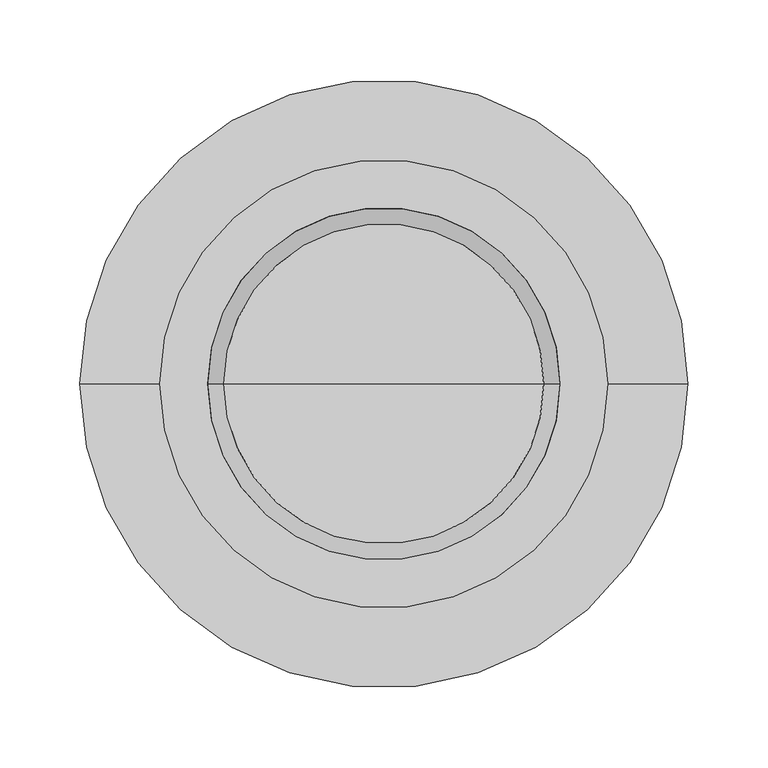
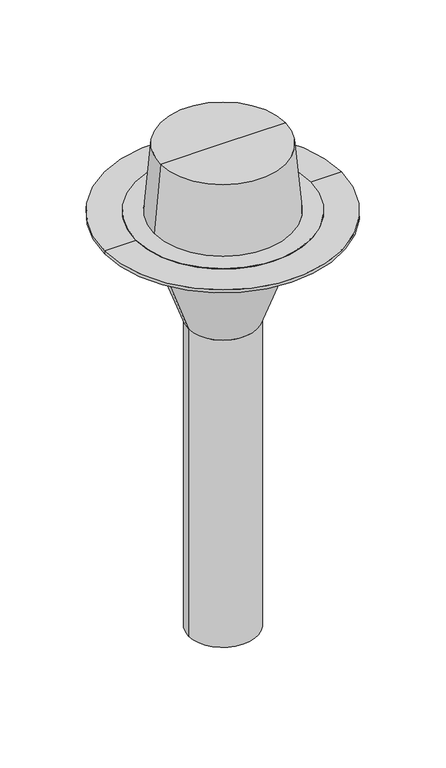
"""IFC4 building model written with IfcOpenShell, lengths in millimetres: proxy geometry, TN_Воронка ТехноНИКОЛЬ ЭКО : Воронка ТехноНИКОЛЬ ЭКО с обжимным фланцем Ø110х700мм."""

import ifcopenshell
import ifcopenshell.guid

model = None  # the IFC model being written
_history = None  # IfcOwnerHistory: only IFC2X3 demands one
_inside = {}  # id of a spatial element -> (the spatial element, [elements in it])
_under = {}  # id of a project, library or spatial element -> (it, [spatial elements below it])
_declared = {}  # id of a project -> (the project, [libraries it declares])
_typed = {}  # id of a type object -> (the type object, [elements of that type])
_made_of = {}  # id of a material, layer set ... -> (it, [elements and type objects made of it])


def new_model(schema):
    """Start an empty IFC model of exactly this schema.

    Asked for "IFC4X3", IfcOpenShell would pick the latest addendum, in which some entities
    have other attributes; the version numbers below select the first issue.
    IFC2X3 requires an IfcOwnerHistory on every rooted entity: one is made here for all.
    """
    global model, _history
    if schema == "IFC4X3":
        model = ifcopenshell.file(schema_version=(4, 3, 0, 0))
    else:
        model = ifcopenshell.file(schema=schema)
    _inside.clear()
    _under.clear()
    _declared.clear()
    _typed.clear()
    _made_of.clear()
    _history = None
    if model.schema == "IFC2X3":
        org = make("IfcOrganization", Name="unknown")
        user = make(
            "IfcPersonAndOrganization",
            ThePerson=make("IfcPerson", FamilyName="unknown"),
            TheOrganization=org,
        )
        app = make(
            "IfcApplication",
            ApplicationDeveloper=org,
            Version="unknown",
            ApplicationFullName="unknown",
            ApplicationIdentifier="unknown",
        )
        _history = make(
            "IfcOwnerHistory",
            OwningUser=user,
            OwningApplication=app,
            ChangeAction="ADDED",
            CreationDate=0,
        )
    return model


def make(cls, **values):
    """One entity of the class cls with the attributes given. An attribute that is None is left unset."""
    return model.create_entity(
        cls, **{name: value for name, value in values.items() if value is not None}
    )


def rooted(cls, **values):
    """An entity with a GlobalId (a new one), such as an element, a storey or a relation."""
    return make(cls, GlobalId=ifcopenshell.guid.new(), OwnerHistory=_history, **values)


def si_unit(unit_type, name, prefix=None):
    """IfcSIUnit, for example si_unit("LENGTHUNIT", "METRE", prefix="MILLI")."""
    return make("IfcSIUnit", UnitType=unit_type, Prefix=prefix, Name=name)


def assignment(units):
    """IfcUnitAssignment: the units of a project."""
    return None if units is None else make("IfcUnitAssignment", Units=units)


def point(xyz):
    """IfcCartesianPoint."""
    return None if xyz is None else make("IfcCartesianPoint", Coordinates=xyz)


def direction(xyz):
    """IfcDirection."""
    return None if xyz is None else make("IfcDirection", DirectionRatios=xyz)


def frame(location, z_axis=None, x_axis=None):
    """IfcAxis2Placement3D, a coordinate frame: its origin and axes. An axis left out is left unset."""
    return make(
        "IfcAxis2Placement3D",
        Location=point(location),
        Axis=direction(z_axis),
        RefDirection=direction(x_axis),
    )


def frame_2d(location, x_axis=None):
    """IfcAxis2Placement2D, a coordinate frame in the plane: its origin and x axis."""
    return make(
        "IfcAxis2Placement2D", Location=point(location), RefDirection=direction(x_axis)
    )


def origin():
    """The frame at (0, 0, 0) with its axes left unset."""
    return frame((0.0, 0.0, 0.0))


def origin_with_axes():
    """The frame at (0, 0, 0) with the z axis (0, 0, 1) and the x axis (1, 0, 0) written out."""
    return frame((0.0, 0.0, 0.0), z_axis=(0.0, 0.0, 1.0), x_axis=(1.0, 0.0, 0.0))


def origin_2d():
    """The frame at (0, 0) in the plane with its x axis left unset."""
    return frame_2d((0.0, 0.0))


def place(relative_to, where):
    """IfcLocalPlacement: puts the frame where relative to a parent placement (None: the world)."""
    return make(
        "IfcLocalPlacement", PlacementRelTo=relative_to, RelativePlacement=where
    )


def context(
    kind, dimensions, precision=None, world=None, true_north=None, identifier=None
):
    """IfcGeometricRepresentationContext, for example the 3D "Model" context."""
    return make(
        "IfcGeometricRepresentationContext",
        ContextIdentifier=identifier,
        ContextType=kind,
        CoordinateSpaceDimension=dimensions,
        Precision=precision,
        WorldCoordinateSystem=world,
        TrueNorth=true_north,
    )


def project(units=None, contexts=None):
    """IfcProject with its units and contexts."""
    return rooted(
        "IfcProject",
        Name="project",
        RepresentationContexts=contexts,
        UnitsInContext=assignment(units),
    )


def spatial(cls, under=None, at=None, **own):
    """A site, building, storey or space (cls), placed at a placement, below another one or the project."""
    s = rooted(cls, ObjectPlacement=at, **own)
    if under is not None:
        _under.setdefault(under.id(), (under, []))[1].append(s)
    return s


def polyline(points):
    """IfcPolyline through the points."""
    return make("IfcPolyline", Points=[point(p) for p in points])


def circle_curve(where, radius):
    """IfcCircle in the frame where."""
    return make("IfcCircle", Position=where, Radius=radius)


def trimmed(basis, trim1, trim2, sense, master):
    """IfcTrimmedCurve: the piece of a basis curve between two trims."""
    return make(
        "IfcTrimmedCurve",
        BasisCurve=basis,
        Trim1=trim1,
        Trim2=trim2,
        SenseAgreement=sense,
        MasterRepresentation=master,
    )


def segment(curve, same_sense, transition):
    """IfcCompositeCurveSegment."""
    return make(
        "IfcCompositeCurveSegment",
        Transition=transition,
        SameSense=same_sense,
        ParentCurve=curve,
    )


def composite_curve(segments, self_intersect=None):
    """IfcCompositeCurve: segments joined end to end."""
    return make("IfcCompositeCurve", Segments=segments, SelfIntersect=self_intersect)


def outline(outer, holes=None, kind="AREA"):
    """IfcArbitraryClosedProfileDef: a profile drawn as a closed curve; with holes, ...WithVoids."""
    if holes is None:
        return make("IfcArbitraryClosedProfileDef", ProfileType=kind, OuterCurve=outer)
    return make(
        "IfcArbitraryProfileDefWithVoids",
        ProfileType=kind,
        OuterCurve=outer,
        InnerCurves=holes,
    )


def extrude(swept, where, along, depth):
    """IfcExtrudedAreaSolid: the profile swept, set in the frame where, extruded along a direction by depth."""
    return make(
        "IfcExtrudedAreaSolid",
        SweptArea=swept,
        Position=where,
        ExtrudedDirection=direction(along),
        Depth=depth,
    )


def shape(context_of_items, identifier, shape_type, items):
    """IfcShapeRepresentation: the items that make up one representation, for example the "Body"."""
    return make(
        "IfcShapeRepresentation",
        ContextOfItems=context_of_items,
        RepresentationIdentifier=identifier,
        RepresentationType=shape_type,
        Items=items,
    )


def source(mapping_origin, context_of_items, identifier, shape_type, items):
    """IfcRepresentationMap: a shape defined once, which mapped items show again and again."""
    return make(
        "IfcRepresentationMap",
        MappingOrigin=mapping_origin,
        MappedRepresentation=shape(context_of_items, identifier, shape_type, items),
    )


def transform(
    local_origin,
    x_axis=None,
    y_axis=None,
    z_axis=None,
    scale=None,
    scale2=None,
    scale3=None,
    uniform=True,
):
    """IfcCartesianTransformationOperator3D, or its non-uniform kind. x_axis, y_axis, z_axis: its Axis1, 2, 3."""
    if uniform:
        return make(
            "IfcCartesianTransformationOperator3D",
            Axis1=direction(x_axis),
            Axis2=direction(y_axis),
            LocalOrigin=point(local_origin),
            Scale=scale,
            Axis3=direction(z_axis),
        )
    return make(
        "IfcCartesianTransformationOperator3DnonUniform",
        Axis1=direction(x_axis),
        Axis2=direction(y_axis),
        LocalOrigin=point(local_origin),
        Scale=scale,
        Axis3=direction(z_axis),
        Scale2=scale2,
        Scale3=scale3,
    )


def mapped(mapping_source, mapping_target):
    """IfcMappedItem: shows the shape of a source again, moved by a transform."""
    return make(
        "IfcMappedItem", MappingSource=mapping_source, MappingTarget=mapping_target
    )


def made_of(thing, what):
    """Note that an element or type object is made of a material, layer set ...; save() writes the relation."""
    if what is not None:
        _made_of.setdefault(what.id(), (what, []))[1].append(thing)
    return thing


def element(
    cls,
    number,
    at=None,
    inside=None,
    cuts=None,
    type_object=None,
    material=None,
    context=None,
    identifier="Body",
    shape_type=None,
    held_by="IfcProductDefinitionShape",
    body=None,
    shapes=None,
    **own,
):
    """One element of the class cls, such as IfcWall. Its Tag is "e" and its number.

    at: its placement. inside: the storey or other place that contains it. cuts: it is an
    opening in that element (IfcRelVoidsElement). A single representation is given by context,
    identifier, shape_type and body (its items); several are given by shapes. held_by: the class
    of the entity that holds the representations. save() writes the other relations.
    """
    e = rooted(cls, Tag="e%d" % number, ObjectPlacement=at, **own)
    if body is not None:
        shapes = [shape(context, identifier, shape_type, body)]
    if shapes is not None:
        e.Representation = make(held_by, Representations=shapes)
    if inside is not None:
        _inside.setdefault(inside.id(), (inside, []))[1].append(e)
    if cuts is not None:
        rooted(
            "IfcRelVoidsElement", RelatingBuildingElement=cuts, RelatedOpeningElement=e
        )
    if type_object is not None:
        _typed.setdefault(type_object.id(), (type_object, []))[1].append(e)
    return made_of(e, material)


def aggregate(whole, parts):
    """IfcRelAggregates: a whole, such as a stair, and the parts it consists of."""
    return rooted("IfcRelAggregates", RelatingObject=whole, RelatedObjects=parts)


def save(model, path):
    """Write the relations noted so far, then the file.

    IfcRelAggregates (storeys below a building ...), IfcRelContainedInSpatialStructure (elements
    in a storey), IfcRelDefinesByType, IfcRelAssociatesMaterial and IfcRelDeclares: one each for
    every whole, place, type object, material and project.
    """
    for whole, parts in _under.values():
        aggregate(whole, parts)
    for where, things in _inside.values():
        rooted(
            "IfcRelContainedInSpatialStructure",
            RelatedElements=things,
            RelatingStructure=where,
        )
    for kind, things in _typed.values():
        rooted("IfcRelDefinesByType", RelatedObjects=things, RelatingType=kind)
    for what, things in _made_of.values():
        rooted("IfcRelAssociatesMaterial", RelatedObjects=things, RelatingMaterial=what)
    for by, libraries in _declared.values():
        rooted("IfcRelDeclares", RelatingContext=by, RelatedDefinitions=libraries)
    model.write(path)


def plane_surface(at):
    """IfcPlane: the flat surface through the origin of the frame at, square to its z axis."""
    return make("IfcPlane", Position=at)


def cylinder_surface(at, radius):
    """IfcCylindricalSurface: all points at the distance radius from the z axis of the frame at."""
    return make("IfcCylindricalSurface", Position=at, Radius=radius)


def revolved_surface(curve, axis_point, axis_direction):
    """IfcSurfaceOfRevolution: the curve turned about the line through axis_point along axis_direction."""
    return make(
        "IfcSurfaceOfRevolution",
        SweptCurve=make("IfcArbitraryOpenProfileDef", ProfileType="CURVE", Curve=curve),
        AxisPosition=make("IfcAxis1Placement", Location=point(axis_point), Axis=direction(axis_direction)),
    )


def advanced_brep(points, edges, surfaces, faces):
    """IfcAdvancedBrep: a solid bounded by faces that lie on surfaces and meet in shared edges.

    An edge is (start, end): straight between two places in points (the first is 0);
    or (start, end, curve); or (start, end, curve, False) where it runs against its curve.
    A face is (place in surfaces, loops), or (place, loops, False) where it looks against
    its surface's normal. A loop lists edges by number (the first is 1), with a minus sign
    where the edge is run from its end to its start. The first loop is the outer one.
    """
    corners = [point(p) for p in points]
    vertices = [make("IfcVertexPoint", VertexGeometry=c) for c in corners]
    made = []
    for start, end, *more in edges:
        made.append(
            make(
                "IfcEdgeCurve",
                EdgeStart=vertices[start],
                EdgeEnd=vertices[end],
                EdgeGeometry=more[0] if more else make("IfcPolyline", Points=[corners[start], corners[end]]),
                SameSense=more[1] if len(more) > 1 else True,
            )
        )
    hull = []
    for where, loops, *sense in faces:
        bounds = []
        for j, loop in enumerate(loops):
            ring = [make("IfcOrientedEdge", EdgeElement=made[abs(k) - 1], Orientation=k > 0) for k in loop]
            bounds.append(
                make(
                    "IfcFaceOuterBound" if j == 0 else "IfcFaceBound",
                    Bound=make("IfcEdgeLoop", EdgeList=ring),
                    Orientation=True,
                )
            )
        hull.append(make("IfcAdvancedFace", Bounds=bounds, FaceSurface=surfaces[where], SameSense=sense[0] if sense else True))
    return make("IfcAdvancedBrep", Outer=make("IfcClosedShell", CfsFaces=hull))


def specialty_equipment_711f7c63(model_context):
    return source(origin(), model_context, "Body", "SolidModel", [
        advanced_brep(
        [(0.0, 0.0, 0.0), (-110.0556416, 0.0, 0.0), (110.0556416, 0.0, 0.0), (100.0, 0.0, 115.0), (-100.0, 0.0, 115.0), (0.0, 0.0, 115.0)],
        [
            (0, 1),
            (1, 2, circle_curve(frame((0.0, 0.0, 0.0), z_axis=(0.0, 0.0, -1.0), x_axis=(-1.0, 0.0, 0.0)), 110.0556416)),
            (2, 0),
            (2, 1, circle_curve(frame((0.0, 0.0, 0.0), z_axis=(0.0, 0.0, -1.0), x_axis=(-1.0, 0.0, 0.0)), 110.0556416)),
            (3, 4, circle_curve(frame((0.0, 0.0, 115.0), z_axis=(0.0, 0.0, 1.0), x_axis=(-1.0, 0.0, 0.0)), 100.0)),
            (4, 5),
            (5, 3),
            (4, 3, circle_curve(frame((0.0, 0.0, 115.0), z_axis=(0.0, 0.0, 1.0), x_axis=(-1.0, 0.0, 0.0)), 100.0)),
            (1, 4),
            (3, 2),
        ],
        [
            plane_surface(frame((0.0, 0.0, 0.0), z_axis=(0.0, 0.0, -1.0), x_axis=(-1.0, 0.0, 0.0))),
            plane_surface(frame((0.0, 0.0, 115.0), z_axis=(0.0, 0.0, 1.0), x_axis=(-1.0, 0.0, 0.0))),
            revolved_surface(polyline([(-100.0, 0.0, 115.0), (-110.0556416, 0.0, 0.0)]), (0.0, 0.0, 0.0), (0.0, 0.0, -1.0)),
        ],
        [
            (0, [[1, 2, 3]]),
            (0, [[-3, 4, -1]]),
            (1, [[5, 6, 7]]),
            (1, [[8, -7, -6]]),
            (2, [[-2, 9, -5, 10]]),
            (2, [[-4, -10, -8, -9]]),
        ],
    ),
        extrude(outline(composite_curve([segment(trimmed(circle_curve(origin_2d(), 140.0), [point((-140.0, 0.0))], [point((140.0, 0.0))], False, "CARTESIAN"), True, "CONTINUOUS"), segment(trimmed(circle_curve(origin_2d(), 140.0), [point((140.0, 0.0))], [point((-140.0, 0.0))], False, "CARTESIAN"), True, "CONTINUOUS")], self_intersect=False), holes=[composite_curve([segment(trimmed(circle_curve(origin_2d(), 110.0556416), [point((-110.0556416, 0.0))], [point((110.0556416, 0.0))], True, "CARTESIAN"), True, "CONTINUOUS"), segment(trimmed(circle_curve(origin_2d(), 110.0556416), [point((110.0556416, 0.0))], [point((-110.0556416, 0.0))], True, "CARTESIAN"), True, "CONTINUOUS")], self_intersect=False)]), origin_with_axes(), (0.0, 0.0, 1.0), 1.0),
        advanced_brep(
        [(0.0, 0.0, -700.0), (-55.0, 0.0, -700.0), (55.0, 0.0, -700.0), (190.0, 0.0, 0.0), (-190.0, 0.0, 0.0), (-83.890873, 0.0, 0.0), (83.890873, 0.0, 0.0), (190.0, 0.0, -5.0), (-190.0, 0.0, -5.0), (93.890873, 0.0, -5.0), (-93.890873, 0.0, -5.0), (55.0, 0.0, -179.9935725), (-55.0, 0.0, -179.9935725), (-93.890873, 0.0, -71.109127), (93.890873, 0.0, -71.109127), (81.9669914, 0.0, -74.7632135), (-81.9669914, 0.0, -74.7632135), (0.0, 0.0, -74.7632135), (83.890873, 0.0, -69.3768397), (-83.890873, 0.0, -69.3768397)],
        [
            (0, 1),
            (1, 2, circle_curve(frame((0.0, 0.0, -700.0), z_axis=(0.0, 0.0, -1.0), x_axis=(-1.0, 0.0, 0.0)), 55.0)),
            (2, 0),
            (2, 1, circle_curve(frame((0.0, 0.0, -700.0), z_axis=(0.0, 0.0, -1.0), x_axis=(-1.0, 0.0, 0.0)), 55.0)),
            (3, 4, circle_curve(frame((0.0, 0.0, 0.0), z_axis=(0.0, 0.0, 1.0), x_axis=(-1.0, 0.0, 0.0)), 190.0)),
            (4, 5),
            (5, 6, circle_curve(frame((0.0, 0.0, 0.0), z_axis=(0.0, 0.0, -1.0), x_axis=(-1.0, 0.0, 0.0)), 83.890873)),
            (6, 3),
            (4, 3, circle_curve(frame((0.0, 0.0, 0.0), z_axis=(0.0, 0.0, 1.0), x_axis=(-1.0, 0.0, 0.0)), 190.0)),
            (6, 5, circle_curve(frame((0.0, 0.0, 0.0), z_axis=(0.0, 0.0, -1.0), x_axis=(-1.0, 0.0, 0.0)), 83.890873)),
            (7, 8, circle_curve(frame((0.0, 0.0, -5.0), z_axis=(0.0, 0.0, 1.0), x_axis=(-1.0, 0.0, 0.0)), 190.0)),
            (8, 4),
            (3, 7),
            (8, 7, circle_curve(frame((0.0, 0.0, -5.0), z_axis=(0.0, 0.0, 1.0), x_axis=(-1.0, 0.0, 0.0)), 190.0)),
            (9, 10, circle_curve(frame((0.0, 0.0, -5.0), z_axis=(0.0, 0.0, 1.0), x_axis=(-1.0, 0.0, 0.0)), 93.890873)),
            (10, 8),
            (7, 9),
            (10, 9, circle_curve(frame((0.0, 0.0, -5.0), z_axis=(0.0, 0.0, 1.0), x_axis=(-1.0, 0.0, 0.0)), 93.890873)),
            (11, 12, circle_curve(frame((0.0, 0.0, -179.9935725), z_axis=(0.0, 0.0, 1.0), x_axis=(-1.0, 0.0, 0.0)), 55.0)),
            (12, 13),
            (13, 14, circle_curve(frame((0.0, 0.0, -71.109127), z_axis=(0.0, 0.0, -1.0), x_axis=(-1.0, 0.0, 0.0)), 93.890873)),
            (14, 11),
            (12, 11, circle_curve(frame((0.0, 0.0, -179.9935725), z_axis=(0.0, 0.0, 1.0), x_axis=(-1.0, 0.0, 0.0)), 55.0)),
            (14, 13, circle_curve(frame((0.0, 0.0, -71.109127), z_axis=(0.0, 0.0, -1.0), x_axis=(-1.0, 0.0, 0.0)), 93.890873)),
            (1, 12),
            (11, 2),
            (15, 16, circle_curve(frame((0.0, 0.0, -74.7632135), z_axis=(0.0, 0.0, 1.0), x_axis=(-1.0, 0.0, 0.0)), 81.9669914)),
            (16, 17),
            (17, 15),
            (16, 15, circle_curve(frame((0.0, 0.0, -74.7632135), z_axis=(0.0, 0.0, 1.0), x_axis=(-1.0, 0.0, 0.0)), 81.9669914)),
            (18, 19, circle_curve(frame((0.0, 0.0, -69.3768397), z_axis=(0.0, 0.0, 1.0), x_axis=(-1.0, 0.0, 0.0)), 83.890873)),
            (19, 16),
            (15, 18),
            (19, 18, circle_curve(frame((0.0, 0.0, -69.3768397), z_axis=(0.0, 0.0, 1.0), x_axis=(-1.0, 0.0, 0.0)), 83.890873)),
            (5, 19),
            (18, 6),
            (13, 10),
            (9, 14),
        ],
        [
            plane_surface(frame((0.0, 0.0, -700.0), z_axis=(0.0, 0.0, -1.0), x_axis=(-1.0, 0.0, 0.0))),
            plane_surface(frame((0.0, 0.0, 0.0), z_axis=(0.0, 0.0, 1.0), x_axis=(-1.0, 0.0, 0.0))),
            cylinder_surface(frame((0.0, 0.0, 0.0), z_axis=(0.0, 0.0, -1.0), x_axis=(-1.0, 0.0, 0.0)), 190.0),
            plane_surface(frame((0.0, 0.0, -5.0), z_axis=(0.0, 0.0, -1.0), x_axis=(-1.0, 0.0, 0.0))),
            revolved_surface(polyline([(-93.890873, 0.0, -71.109127), (-55.0, 0.0, -179.9935725)]), (0.0, 0.0, 0.0), (0.0, 0.0, -1.0)),
            cylinder_surface(frame((0.0, 0.0, 0.0), z_axis=(0.0, 0.0, -1.0), x_axis=(-1.0, 0.0, 0.0)), 55.0),
            plane_surface(frame((0.0, 0.0, -74.7632135), z_axis=(0.0, 0.0, 1.0), x_axis=(-1.0, 0.0, 0.0))),
            revolved_surface(polyline([(-81.9669914, 0.0, -74.7632135), (-83.890873, 0.0, -69.3768397)]), (0.0, 0.0, 0.0), (0.0, 0.0, -1.0)),
            revolved_surface(polyline([(-83.890873, 0.0, -69.3768397), (-83.890873, 0.0, 0.0)]), (0.0, 0.0, 0.0), (0.0, 0.0, -1.0)),
            cylinder_surface(frame((0.0, 0.0, 0.0), z_axis=(0.0, 0.0, -1.0), x_axis=(-1.0, 0.0, 0.0)), 93.890873),
        ],
        [
            (0, [[1, 2, 3]]),
            (0, [[-3, 4, -1]]),
            (1, [[5, 6, 7, 8]]),
            (1, [[9, -8, 10, -6]]),
            (2, [[11, 12, -5, 13]]),
            (2, [[14, -13, -9, -12]]),
            (3, [[15, 16, -11, 17]]),
            (3, [[18, -17, -14, -16]]),
            (4, [[19, 20, 21, 22]]),
            (4, [[23, -22, 24, -20]]),
            (5, [[-2, 25, -19, 26]]),
            (5, [[-4, -26, -23, -25]]),
            (6, [[27, 28, 29]]),
            (6, [[30, -29, -28]]),
            (7, [[31, 32, -27, 33]]),
            (7, [[34, -33, -30, -32]]),
            (8, [[-7, 35, -31, 36]]),
            (8, [[-10, -36, -34, -35]]),
            (9, [[-21, 37, -15, 38]]),
            (9, [[-24, -38, -18, -37]]),
        ],
    ),
    ])


if __name__ == "__main__":
    model = new_model("IFC4")
    model_context = context("Model", 3, world=origin())
    ifc_project = project(units=[si_unit("LENGTHUNIT", "METRE", prefix="MILLI")], contexts=[model_context])
    site = spatial("IfcSite", under=ifc_project)
    building = spatial("IfcBuilding", under=site)
    placement = place(None, origin())
    specialty_equipment_shape = specialty_equipment_711f7c63(model_context)
    element("IfcBuildingElementProxy", 1, Name="TN_Воронка ТехноНИКОЛЬ ЭКО : Воронка ТехноНИКОЛЬ ЭКО с обжимным фланцем Ø110х700мм", ObjectType="TN_Воронка ТехноНИКОЛЬ ЭКО : Воронка ТехноНИКОЛЬ ЭКО с обжимным фланцем Ø110х700мм", at=placement, inside=building, context=model_context, shape_type="MappedRepresentation", body=[
        mapped(specialty_equipment_shape, transform((0.0, 0.0, 0.0), x_axis=(1.0, 0.0, 0.0), y_axis=(0.0, 1.0, 0.0), z_axis=(0.0, 0.0, 1.0))),
    ])
    save(model, "model.ifc")

# Revit data of these elements
# Type "TN_Воронка ТехноНИКОЛЬ ЭКО : Воронка ТехноНИКОЛЬ ЭКО с обжимным фланцем Ø110х700мм"
#   ADSK_Группирование = "Комплектующие и воронки"
#   Description = "Воронки ТехноНИКОЛЬ для водоотвода с поверхности кровли в системах внутреннего водостока. Изготавливается из смеси полимеров, устойчивых к атмосферным воздействиям и УФ излучению."
#   Manufacturer = "ТехноНИКОЛЬ"
#   URL = "https://nav.tn.ru/catalog/krovlya/vodostochnaya-sistema/voronka-tekhnonikol-s-obzhimnym-flantsem-/?sphrase_id=460380"
#   ADSK_Примечание = ""
#   ADSK_Обозначение = "ТехноНИКОЛЬ"
#   ADSK_Наименование = "Воронка ТехноНИКОЛЬ ЭКО с обжимным фланцем Ø110х700мм"
#   ADSK_Масса_Текст = ""
#   ADSK_Марка = ""
#   ADSK_Код изделия = "52494"
#   ADSK_Завод-изготовитель = "ТехноНИКОЛЬ"
#   ADSK_Единица измерения = "шт."
#   ADSK_Группирование = "Комплектующие и воронки"
#   ADSK_URL страницы изделия = "https://nav.tn.ru/catalog/krovlya/vodostochnaya-sistema/voronka-tekhnonikol-s-obzhimnym-flantsem-/?sphrase_id=460380"
#   ADSK_URL документации изделия = ""
#   Радиус = 55 mm
#   Пропускная способность = 7.8 L/s
#   Монтажный диаметр = 110 mm
#   Длина расчетная [instance default] = 700 mm
#   Длина отвода [instance default] = 700 mm
#   ADSK_Масса = 2
#   ADSK_Количество = 1
#   Видимость_Листоуловитель [instance default] = yes
#   Материал_Фланец = TN_Фланец_Синий
#   Материал_Корпус = TN_ПВХ_Черный
#   Default Elevation = 0
# Element 1 (IfcBuildingElementProxy, "TN_Воронка ТехноНИКОЛЬ ЭКО : Воронка ТехноНИКОЛЬ ЭКО с обжимным фланцем Ø110х700мм")
#   Materials on its faces: "TN_ПВХ_Черный", "TN_Фланец_Синий"
# Materials
#   "TN_Фланец_Синий": class "Типовые", colour RGB 0 15 119, transparency 0, Cost = 0
#   "TN_ПВХ_Черный": class "Типовые", colour RGB 48 48 48, transparency 0, Cost = 0
